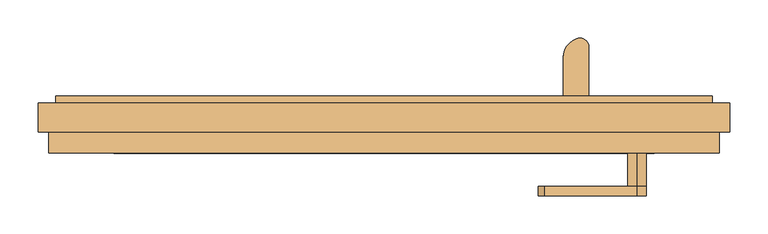
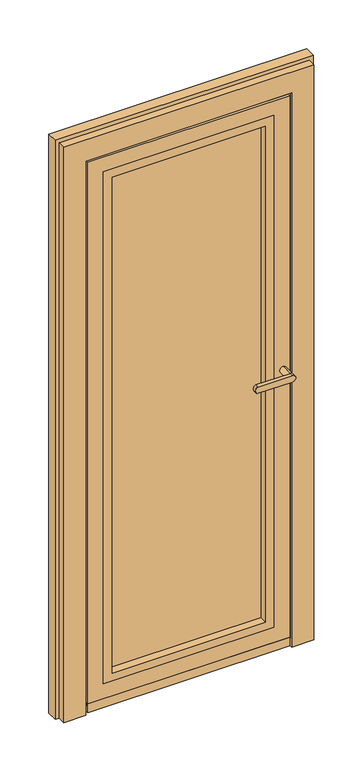
"""IFC4 building model written with IfcOpenShell, lengths in millimetres: door geometry, Schueco_FWS_ADS-75-SimplySmart_out_Family-01 : FWS SI insert unit."""

from ifc_helpers import new_model, si_unit, point, frame, frame_2d, origin, place, context, project, spatial, polyline, circle_curve, ellipse_curve, trimmed, segment, composite_curve, outline, extrude, faceted_brep, source, transform, mapped, element, save
from ifc_brep_helpers import plane_surface, cylinder_surface, extruded_surface, advanced_brep


def door_c76f04af(model_context):
    return source(origin(), model_context, "Body", "SolidModel", [
        extrude(outline(composite_curve([segment(polyline([(235.3326764, 8.9997177), (235.3326764, 59.1618682)]), True, "CONTINUOUS"), segment(trimmed(circle_curve(frame_2d((262.5110941, 59.1618682)), 27.1784177), [point((235.3326764, 59.1618682))], [point((252.9739985, 84.6120194))], False, "CARTESIAN"), True, "CONTINUOUS"), segment(trimmed(circle_curve(frame_2d((257.0514995, 73.7310321)), 11.6198924), [point((252.9739985, 84.6120194))], [point((268.6713919, 73.7310321))], False, "CARTESIAN"), True, "CONTINUOUS"), segment(polyline([(268.6713919, 73.7310321), (268.6713919, 8.9997177), (235.3326764, 8.9997177)]), True, "CONTINUOUS")], self_intersect=False)), frame((0.0, 0.0, 2040.9218203), z_axis=(0.0, 0.0, 1.0), x_axis=(1.0, 0.0, 0.0)), (0.0, 0.0, 1.0), 4.0),
        extrude(outline(polyline([(235.3326764, 12.9997177), (268.6713919, 12.9997177), (268.6713919, 8.9997177), (235.3326764, 8.9997177), (235.3326764, 12.9997177)])), frame((0.0, 0.0, 2010.9218203), z_axis=(0.0, 0.0, 1.0), x_axis=(1.0, 0.0, 0.0)), (0.0, 0.0, 1.0), 30.0),
        extrude(outline(polyline([(235.3326764, 12.9997177), (268.6713919, 12.9997177), (268.6713919, 8.9997177), (235.3326764, 8.9997177), (235.3326764, 12.9997177)])), frame((0.0, 0.0, 49.9218203), z_axis=(0.0, 0.0, 1.0), x_axis=(1.0, 0.0, 0.0)), (0.0, 0.0, 1.0), 30.0),
        extrude(outline(composite_curve([segment(polyline([(235.3326764, 8.9997177), (235.3326764, 59.1618682)]), True, "CONTINUOUS"), segment(trimmed(circle_curve(frame_2d((262.5110941, 59.1618682)), 27.1784177), [point((235.3326764, 59.1618682))], [point((252.9739985, 84.6120194))], False, "CARTESIAN"), True, "CONTINUOUS"), segment(trimmed(circle_curve(frame_2d((257.0514995, 73.7310321)), 11.6198924), [point((252.9739985, 84.6120194))], [point((268.6713919, 73.7310321))], False, "CARTESIAN"), True, "CONTINUOUS"), segment(polyline([(268.6713919, 73.7310321), (268.6713919, 8.9997177), (235.3326764, 8.9997177)]), True, "CONTINUOUS")], self_intersect=False)), frame((0.0, 0.0, 45.9218203), z_axis=(0.0, 0.0, 1.0), x_axis=(1.0, 0.0, 0.0)), (0.0, 0.0, 1.0), 4.0),
        advanced_brep(
        [(264.717076, 57.5977179, 2040.9218203), (239.282924, 72.2821425, 2040.9218203), (264.717076, 57.5977179, 49.9218203), (239.282924, 72.2821425, 49.9218203)],
        [
            (0, 1, ellipse_curve(frame((252.0, 64.9399302, 2040.9218203), z_axis=(0.0, 0.0, 1.0000000000000002), x_axis=(0.5000002582658958, 0.866025254674503, 0.0)), 21.5840887, 14.6844171)),
            (1, 0, ellipse_curve(frame((252.0, 64.9399302, 2040.9218203), z_axis=(0.0, 0.0, 1.0000000000000002), x_axis=(0.5000002582658958, 0.866025254674503, 0.0)), 21.5840887, 14.6844171)),
            (2, 3, ellipse_curve(frame((252.0, 64.9399302, 49.9218203), z_axis=(0.0, 0.0, -1.0000000000000002), x_axis=(-0.866025254674503, 0.5000002582658958, 0.0)), 14.6844171, 21.5840887)),
            (3, 2, ellipse_curve(frame((252.0, 64.9399302, 49.9218203), z_axis=(0.0, 0.0, -1.0000000000000002), x_axis=(-0.866025254674503, 0.5000002582658958, 0.0)), 14.6844171, 21.5840887)),
            (0, 2),
            (3, 1),
        ],
        [
            plane_surface(frame((239.282924, 72.2821425, 2040.9218203), z_axis=(0.0, 0.0, 1.0000000000000002), x_axis=(0.5000002582658958, 0.866025254674503, 0.0))),
            plane_surface(frame((239.282924, 72.2821425, 49.9218203), z_axis=(0.0, 0.0, -1.0000000000000002), x_axis=(-0.5000002582658958, -0.866025254674503, 0.0))),
            extruded_surface(trimmed(ellipse_curve(frame((252.0, 64.9399302, 49.9218203), z_axis=(0.0, 0.0, -1.0000000000000002), x_axis=(-0.866025254674503, 0.5000002582658958, 0.0)), 14.6844171, 21.5840887), [point((239.282924, 72.2821425, 49.9218203))], [point((264.717076, 57.5977179, 49.9218203))], True, "CARTESIAN"), (0.0, 0.0, -1991.0), 1991.0),
            extruded_surface(trimmed(ellipse_curve(frame((252.0, 64.9399302, 49.9218203), z_axis=(0.0, 0.0, -1.0000000000000002), x_axis=(-0.866025254674503, 0.5000002582658958, 0.0)), 14.6844171, 21.5840887), [point((264.717076, 57.5977179, 49.9218203))], [point((239.282924, 72.2821425, 49.9218203))], True, "CARTESIAN"), (0.0, 0.0, -1991.0), 1991.0),
        ],
        [
            (0, [[1, 2]]),
            (1, [[3, 4]]),
            (2, [[5, -4, 6, -1]]),
            (3, [[-6, -3, -5, -2]]),
        ],
    ),
        advanced_brep(
        [(332.0, -122.0002518, 1030.9991882), (332.0, -122.0002518, 1054.9764498), (210.3382074, -122.0002518, 1054.9764498), (210.3382074, -122.0002518, 1030.9991882), (332.0, -109.5001648, 1054.9764498), (332.0, -109.5001648, 1030.9991882), (210.3382074, -109.5001648, 1030.9991882), (210.3382074, -109.5001648, 1054.9764498), (332.0, -66.0002823, 1030.9991882), (332.0, -66.0002823, 1054.9764498)],
        [
            (0, 1, circle_curve(frame((332.0, -122.0002518, 1042.987819), z_axis=(0.0, -1.0, 0.0), x_axis=(0.0, 0.0, 1.0)), 11.9886308)),
            (1, 2),
            (2, 3, ellipse_curve(frame((210.3382074, -122.0002518, 1042.987819), z_axis=(0.0, -1.0, 0.0), x_axis=(0.0, 0.0, -1.0)), 11.9886308, 7.9050795)),
            (3, 0),
            (4, 5, circle_curve(frame((332.0, -109.5001648, 1042.987819), z_axis=(0.0, -1.0, 0.0), x_axis=(0.0, 0.0, 1.0)), 11.9886308)),
            (5, 6),
            (6, 7, ellipse_curve(frame((210.3382074, -109.5001648, 1042.987819), z_axis=(0.0, 1.0, 0.0), x_axis=(0.0, 0.0, -1.0)), 11.9886308, 7.9050795)),
            (7, 4),
            (3, 6),
            (5, 0),
            (2, 7),
            (1, 4),
            (5, 4, circle_curve(frame((332.0, -109.5001648, 1042.987819), z_axis=(0.0, -1.0, 0.0), x_axis=(0.0, 0.0, 1.0)), 11.9886308)),
            (8, 9, circle_curve(frame((332.0, -66.0002823, 1042.987819), z_axis=(0.0, 1.0, 0.0), x_axis=(0.0, 0.0, 1.0)), 11.9886308)),
            (9, 8, circle_curve(frame((332.0, -66.0002823, 1042.987819), z_axis=(0.0, 1.0, 0.0), x_axis=(0.0, 0.0, 1.0)), 11.9886308)),
            (8, 5),
            (4, 9),
        ],
        [
            plane_surface(frame((210.3382074, -122.0002518, 1030.9991882), z_axis=(0.0, -1.0, 0.0), x_axis=(-1.0, 0.0, 0.0))),
            plane_surface(frame((210.3382074, -109.5001648, 1030.9991882), z_axis=(0.0, 1.0, 0.0), x_axis=(1.0, 0.0, 0.0))),
            plane_surface(frame((332.0, -122.0002518, 1030.9991882), z_axis=(0.0, 0.0, -1.0), x_axis=(0.0, 1.0, 0.0))),
            extruded_surface(trimmed(ellipse_curve(frame((210.3382074, -109.5001648, 1042.987819), z_axis=(0.0, 1.0, 0.0), x_axis=(0.0, 0.0, -1.0)), 11.9886308, 7.9050795), [point((210.3382074, -109.5001648, 1030.9991882))], [point((210.3382074, -109.5001648, 1054.9764498))], True, "CARTESIAN"), (0.0, 12.500086999999994, 0.0), 12.500086999999994),
            plane_surface(frame((210.3382074, -122.0002518, 1054.9764498), z_axis=(0.0, 0.0, 1.0), x_axis=(0.0, 1.0, 0.0))),
            cylinder_surface(frame((332.0, -109.5001648, 1042.987819), z_axis=(0.0, -1.0, 0.0), x_axis=(0.0, 0.0, 1.0)), 11.9886308),
            plane_surface(frame((332.0, -66.0002823, 1054.9764498), z_axis=(0.0, 1.0, 0.0), x_axis=(-1.0, 0.0, 0.0))),
            cylinder_surface(frame((332.0, -66.0002823, 1042.987819), z_axis=(0.0, -1.0, 0.0), x_axis=(0.0, 0.0, 1.0)), 11.9886308),
        ],
        [
            (0, [[1, 2, 3, 4]]),
            (1, [[5, 6, 7, 8]]),
            (2, [[9, -6, 10, -4]]),
            (3, [[11, -7, -9, -3]]),
            (4, [[12, -8, -11, -2]]),
            (5, [[-10, 13, -12, -1]]),
            (6, [[14, 15]]),
            (7, [[16, -5, 17, -14]]),
            (7, [[-17, -13, -16, -15]]),
        ],
    ),
        extrude(outline(polyline([(94.987819, 300.0), (1999.987819, 300.0), (1999.987819, -300.0), (94.987819, -300.0), (94.987819, 300.0)]), holes=[polyline([(124.987819, -270.0), (1969.987819, -270.0), (1969.987819, 270.0), (124.987819, 270.0), (124.987819, -270.0)])]), frame((0.0, -66.0002823, 0.0), z_axis=(0.0, 1.0, 0.0), x_axis=(0.0, 0.0, 1.0)), (0.0, 0.0, 1.0), 28.0002823),
        faceted_brep([(-355.0, -66.0002823, 2054.987819), (-355.0, -57.5000065, 2054.987819), (-355.0, -57.5000065, 39.987819), (-355.0, -66.0002823, 39.987819), (355.0, -57.5000065, 39.987819), (355.0, -66.0002823, 39.987819), (368.0, -57.5000065, 26.987819), (368.0, -57.5000065, 2067.987819), (-368.0, -57.5000065, 2067.987819), (-368.0, -57.5000065, 26.987819), (355.0, -57.5000065, 2054.987819), (355.0, -66.0002823, 2054.987819), (-300.0, -66.0002823, 94.987819), (-300.0, -66.0002823, 1999.987819), (300.0, -66.0002823, 1999.987819), (300.0, -66.0002823, 94.987819), (-300.0, 0.0, 1999.987819), (-300.0, 0.0, 94.987819), (300.0, 0.0, 94.987819), (300.0, 0.0, 1999.987819), (-268.0, 0.0, 126.987819), (-268.0, 0.0, 1967.987819), (268.0, 0.0, 1967.987819), (268.0, 0.0, 126.987819), (-268.0, 8.9997177, 1967.987819), (-268.0, 8.9997177, 126.987819), (268.0, 8.9997177, 126.987819), (268.0, 8.9997177, 1967.987819), (-387.0, 8.9997177, 7.987819), (-387.0, 8.9997177, 2086.987819), (387.0, 8.9997177, 2086.987819), (387.0, 8.9997177, 7.987819), (-387.0, 0.4997603, 2086.987819), (-387.0, 0.4997603, 7.987819), (387.0, 0.4997603, 7.987819), (387.0, 0.4997603, 2086.987819), (-368.0, 0.4997603, 26.987819), (-368.0, 0.4997603, 2067.987819), (368.0, 0.4997603, 2067.987819), (368.0, 0.4997603, 26.987819)], [[[0, 1, 2, 3]], [[3, 2, 4, 5]], [[6, 7, 8, 9], [2, 1, 10, 4]], [[5, 4, 10, 11]], [[5, 11, 0, 3], [12, 13, 14, 15]], [[16, 13, 12, 17]], [[17, 12, 15, 18]], [[18, 15, 14, 19]], [[18, 19, 16, 17], [20, 21, 22, 23]], [[24, 21, 20, 25]], [[25, 20, 23, 26]], [[26, 23, 22, 27]], [[28, 29, 30, 31], [26, 27, 24, 25]], [[32, 29, 28, 33]], [[33, 28, 31, 34]], [[34, 31, 30, 35]], [[34, 35, 32, 33], [36, 37, 38, 39]], [[8, 37, 36, 9]], [[9, 36, 39, 6]], [[6, 39, 38, 7]], [[11, 10, 1, 0]], [[19, 14, 13, 16]], [[27, 22, 21, 24]], [[35, 30, 29, 32]], [[7, 38, 37, 8]]]),
        extrude(outline(polyline([(300.0, -38.0), (-300.0, -38.0), (-300.0, 0.0), (300.0, 0.0), (300.0, -38.0)])), frame((0.0, 0.0, 94.987819), z_axis=(0.0, 0.0, 1.0), x_axis=(1.0, 0.0, 0.0)), (0.0, 0.0, 1.0), 1905.0),
        extrude(outline(composite_curve([segment(polyline([(-39.1486683, 26.987819), (-17.8439358, 26.987819), (-17.8439358, 3.5881205)]), True, "CONTINUOUS"), segment(trimmed(circle_curve(frame_2d((-28.496302, 19.4783613)), 19.1304119), [point((-17.8439358, 3.5881205))], [point((-39.1486683, 3.5881205))], False, "CARTESIAN"), True, "CONTINUOUS"), segment(polyline([(-39.1486683, 3.5881205), (-39.1486683, 26.987819)]), True, "CONTINUOUS")], self_intersect=False)), frame((-368.0, 0.0, 0.0), z_axis=(1.0, 0.0, 0.0), x_axis=(0.0, 1.0, 0.0)), (0.0, 0.0, 1.0), 736.0),
        extrude(outline(polyline([(-355.0, -66.0002823), (-355.0, -57.5000065), (355.0, -57.5000065), (355.0, -66.0002823), (-355.0, -66.0002823)])), frame((0.0, 0.0, 7.987819), z_axis=(0.0, 0.0, 1.0), x_axis=(1.0, 0.0, 0.0)), (0.0, 0.0, 1.0), 32.0),
        faceted_brep([(430.999943, 8.9997177, 2130.999943), (430.999943, 0.0, 2130.999943), (430.999943, 0.0, 0.0), (430.999943, 8.9997177, 0.0), (-454.0, 0.0, 0.0), (-454.0, 0.0, 2154.0), (454.0, 0.0, 2154.0), (454.0, 0.0, 0.0), (-430.999943, 0.0, 2130.999943), (-430.999943, 0.0, 0.0), (454.0, -38.0, 0.0), (440.0, -38.0, 0.0), (440.0, -66.0002823, 0.0), (361.9999732, -66.0002823, 0.0), (361.9999732, -57.5000065, 0.0), (382.4999732, -57.5000065, 0.0), (382.4999732, 0.4997603, 0.0), (393.9999732, 0.4997603, 0.0), (393.9999732, 8.9997177, 0.0), (-393.9999732, 8.9997177, 0.0), (-430.999943, 8.9997177, 0.0), (-430.999943, 8.9997177, 2130.999943), (393.9999732, 8.9997177, 2093.9999732), (-393.9999732, 8.9997177, 2093.9999732), (361.9999732, -66.0002823, 2061.9999732), (361.9999732, -57.5000065, 2061.9999732), (-361.9999732, -57.5000065, 0.0), (-382.4999732, -57.5000065, 0.0), (-382.4999732, -57.5000065, 2082.4999732), (382.4999732, -57.5000065, 2082.4999732), (-361.9999732, -57.5000065, 2061.9999732), (-440.0, -66.0002823, 0.0), (-361.9999732, -66.0002823, 0.0), (-361.9999732, -66.0002823, 2061.9999732), (440.0, -66.0002823, 2140.0), (-440.0, -66.0002823, 2140.0), (440.0, -38.0, 2140.0), (-454.0, -38.0, 0.0), (-440.0, -38.0, 0.0), (-440.0, -38.0, 2140.0), (454.0, -38.0, 2154.0), (-454.0, -38.0, 2154.0), (-393.9999732, 0.4997603, 0.0), (-382.4999732, 0.4997603, 0.0), (393.9999732, 0.4997603, 2093.9999732), (-393.9999732, 0.4997603, 2093.9999732), (382.4999732, 0.4997603, 2082.4999732), (-382.4999732, 0.4997603, 2082.4999732)], [[[0, 1, 2, 3]], [[4, 5, 6, 7, 2, 1, 8, 9]], [[3, 2, 7, 10, 11, 12, 13, 14, 15, 16, 17, 18]], [[19, 20, 21, 0, 3, 18, 22, 23]], [[24, 25, 14, 13]], [[26, 27, 28, 29, 15, 14, 25, 30]], [[31, 32, 33, 24, 13, 12, 34, 35]], [[34, 12, 11, 36]], [[37, 38, 39, 36, 11, 10, 40, 41]], [[4, 9, 20, 19, 42, 43, 27, 26, 32, 31, 38, 37]], [[20, 9, 8, 21]], [[18, 17, 44, 22]], [[42, 19, 23, 45]], [[32, 26, 30, 33]], [[31, 35, 39, 38]], [[4, 37, 41, 5]], [[6, 40, 10, 7]], [[43, 42, 45, 44, 17, 16, 46, 47]], [[16, 15, 29, 46]], [[27, 43, 47, 28]], [[21, 8, 1, 0]], [[33, 30, 25, 24]], [[35, 34, 36, 39]], [[23, 22, 44, 45]], [[5, 41, 40, 6]], [[47, 46, 29, 28]]]),
    ])


if __name__ == "__main__":
    model = new_model("IFC4")
    model_context = context("Model", 3, world=origin())
    ifc_project = project(units=[si_unit("LENGTHUNIT", "METRE", prefix="MILLI")], contexts=[model_context])
    site = spatial("IfcSite", under=ifc_project)
    building = spatial("IfcBuilding", under=site)
    placement = place(None, origin())
    door_shape = door_c76f04af(model_context)
    element("IfcDoor", 1, ObjectType="Schueco_FWS_ADS-75-SimplySmart_out_Family-01 : FWS SI insert unit", at=placement, inside=building, context=model_context, shape_type="MappedRepresentation", body=[
        mapped(door_shape, transform((0.0, 0.0, 0.0), x_axis=(1.0, 0.0, 0.0), y_axis=(0.0, 1.0, 0.0), z_axis=(0.0, 0.0, 1.0))),
    ])
    save(model, "model.ifc")

# Revit data of these elements
# Type "Schueco_FWS_ADS-75-SimplySmart_out_Family-01 : FWS SI insert unit"
#   Type Mark = "55"
#   __NOTE__ = "Data describes the optimum values of the entire system. The properites of a selected design option have to be determined on an individual basis!"
#   Wind load resistance = "Class C3"
#   Watertightness = "Class E750"
#   Thermal insulation = "Uf = 1.6 W/(m²K)"
#   Sound insulation = "..."
#   Schueco thermal insulation standard = "Highly thermally insulated"
#   Opening type = "Outward-opening, Flush-fitted"
#   Model = "Schueco ADS 75 SimplySmart"
#   Mechanical loading = "..."
#   Maximum leaf width in mm = "1400"
#   Maximum leaf weight in kg = "200"
#   Maximum leaf height in mm = "3000"
#   Material = "Aluminium"
#   Construction Type = "Door, single-leaf, outward-opening"
#   Manufacturer = "Schueco International KG"
#   Long term functionality = "..."
#   Glazing data = "Triple glazing 38mm"
#   Façade insert unit = "yes"
#   Family creation date = "08.2017"
#   Description = "Schueco Aluminium Door System (ADS)"
#   Burglar resistance = "Class RC 2"
#   Areas of use = "Public buildings, Residential buildings, Side entrance"
#   Analytic Construction = "<None>"
#   Air permeability = "Class 4"
#   Width [instance default] = 934.318 mm
#   Leaf opening angle [instance default] = 0.00°
#   IOf_T = 38 mm
#   Height [instance default] = 1907.117 mm
#   Glazing area [instance default] = 0.896401 m²
#   Distance from bottom to handles [instance default] = 1050 mm
#   Clear opening width [instance default] = 750.318 mm
#   Standard threshold = no
#   Low level threshold = yes
#   Handles = yes
#   Glass = none
#   Frame = Alu
#   Fittings = none
# Element 1 (IfcDoor, "Schueco_FWS_ADS-75-SimplySmart_out_Family-01 : FWS SI insert unit")
#   Width = 908 mm
#   Height = 2154 mm
#   Glazing area = 0.986776 m²
#   Clear opening width = 724 mm
#   Materials on its faces: "Alu", "Glass"
# Materials
#   "Alu": class "Glas", colour RGB 140 140 140, transparency 0
#   "Glass": class "Glass", colour RGB 128 128 255, transparency 0.75, Description = "Soda Lime Glass", Cost = 0
